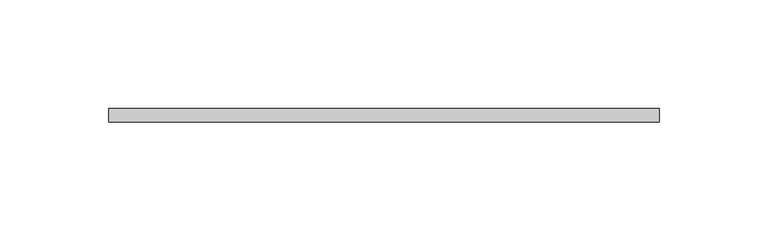
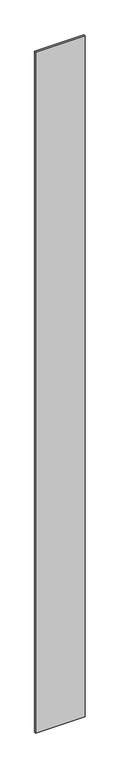
"""IFC4 building model written with IfcOpenShell, lengths in millimetres: proxy geometry, Inner panel1:Inner panel:306176:Inner panel:306176 : Inner panel1:Inner panel:306176:300391:Inner panel:306176:Inner panel:306176 : Inner panel1:Inner panel:306176:300391 : Inner panel1:Inner panel:306176:Inner panel:306176 : Inner panel1:Inner panel:306176:300391:7 : Inner panel1:Inner panel:306176:Inner panel:306176 : Inner panel1:Inner panel:306176:300391:Inner panel:306176:Inner panel:306176 : Inner panel1:Inner panel:306176:300391 : Inner panel1:Inner panel:306176:Inner panel:306176 : Inner panel1:Inner panel:306176:300391:300168."""

from ifc_helpers import new_model, si_unit, frame, origin, place, context, project, spatial, polyline, outline, extrude, source, transform, mapped, element, save


def generic_models_07d8fcdc(model_context):
    return source(origin(), model_context, "Body", "SweptSolid", [
        extrude(outline(polyline([(595962.3515778, -578778.4413841), (595962.3515778, -578772.0913841), (596216.1742239, -578772.0913841), (596216.1742239, -578778.4413841), (595962.3515778, -578778.4413841)])), frame((0.0, 0.0, 25.4), z_axis=(0.0, 0.0, 1.0), x_axis=(1.0, 0.0, 0.0)), (0.0, 0.0, 1.0), 3689.35),
    ])


if __name__ == "__main__":
    model = new_model("IFC4")
    model_context = context("Model", 3, world=origin())
    ifc_project = project(units=[si_unit("LENGTHUNIT", "METRE", prefix="MILLI")], contexts=[model_context])
    site = spatial("IfcSite", under=ifc_project)
    building = spatial("IfcBuilding", under=site)
    placement = place(None, origin())
    generic_models_shape = generic_models_07d8fcdc(model_context)
    element("IfcBuildingElementProxy", 1, Name="Inner panel1:Inner panel:306176:Inner panel:306176 : Inner panel1:Inner panel:306176:300391:Inner panel:306176:Inner panel:306176 : Inner panel1:Inner panel:306176:300391 : Inner panel1:Inner panel:306176:Inner panel:306176 : Inner panel1:Inner panel:306176:300391:7 : Inner panel1:Inner panel:306176:Inner panel:306176 : Inner panel1:Inner panel:306176:300391:Inner panel:306176:Inner panel:306176 : Inner panel1:Inner panel:306176:300391 : Inner panel1:Inner panel:306176:Inner panel:306176 : Inner panel1:Inner panel:306176:300391:300168", ObjectType="Inner panel1:Inner panel:306176:Inner panel:306176 : Inner panel1:Inner panel:306176:300391:Inner panel:306176:Inner panel:306176 : Inner panel1:Inner panel:306176:300391 : Inner panel1:Inner panel:306176:Inner panel:306176 : Inner panel1:Inner panel:306176:300391:7 : Inner panel1:Inner panel:306176:Inner panel:306176 : Inner panel1:Inner panel:306176:300391:Inner panel:306176:Inner panel:306176 : Inner panel1:Inner panel:306176:300391 : Inner panel1:Inner panel:306176:Inner panel:306176 : Inner panel1:Inner panel:306176:300391:300168", at=placement, inside=building, context=model_context, shape_type="MappedRepresentation", body=[
        mapped(generic_models_shape, transform((0.0, 0.0, 0.0), x_axis=(1.0, 0.0, 0.0), y_axis=(0.0, 1.0, 0.0), z_axis=(0.0, 0.0, 1.0))),
    ])
    save(model, "model.ifc")

# Revit data of these elements
# Type "Inner panel1:Inner panel:306176:Inner panel:306176 : Inner panel1:Inner panel:306176:300391:Inner panel:306176:Inner panel:306176 : Inner panel1:Inner panel:306176:300391 : Inner panel1:Inner panel:306176:Inner panel:306176 : Inner panel1:Inner panel:306176:300391:7 : Inner panel1:Inner panel:306176:Inner panel:306176 : Inner panel1:Inner panel:306176:300391:Inner panel:306176:Inner panel:306176 : Inner panel1:Inner panel:306176:300391 : Inner panel1:Inner panel:306176:Inner panel:306176 : Inner panel1:Inner panel:306176:300391:300168"
#   NameOverride = "Inner panel1:Inner panel:306176:Inner panel:306176 : Inner panel1:Inner panel:306176:300391:Inner panel:306176:Inner panel:306176 : Inner panel1:Inner panel:306176:300391 : Inner panel1:Inner panel:306176:Inner panel:306176 : Inner panel1:Inner panel:306176:300391:300168"
#   ObjectTypeOverride = "Inner panel:306176:Inner panel:306176 : Inner panel1:Inner panel:306176:300391 : Inner panel1:Inner panel:306176:Inner panel:306176 : Inner panel1:Inner panel:306176:300391"
#   Reference = "Inner panel"
#   Tag = "300168"
# Element 1 (IfcBuildingElementProxy, "Inner panel1:Inner panel:306176:Inner panel:306176 : Inner panel1:Inner panel:306176:300391:Inner panel:306176:Inner panel:306176 : Inner panel1:Inner panel:306176:300391 : Inner panel1:Inner panel:306176:Inner panel:306176 : Inner panel1:Inner panel:306176:300391:7 : Inner panel1:Inner panel:306176:Inner panel:306176 : Inner panel1:Inner panel:306176:300391:Inner panel:306176:Inner panel:306176 : Inner panel1:Inner panel:306176:300391 : Inner panel1:Inner panel:306176:Inner panel:306176 : Inner panel1:Inner panel:306176:300391:300168")
#   Materials on its faces: "CERAMIC TILE"
# Materials
#   "CERAMIC TILE": class "Generic", colour RGB 87 103 117, transparency 0, Cost = 0
